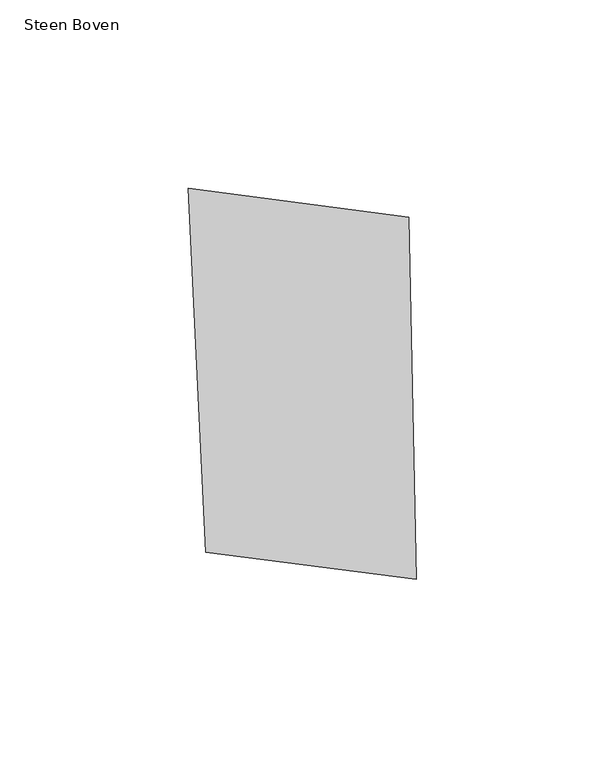
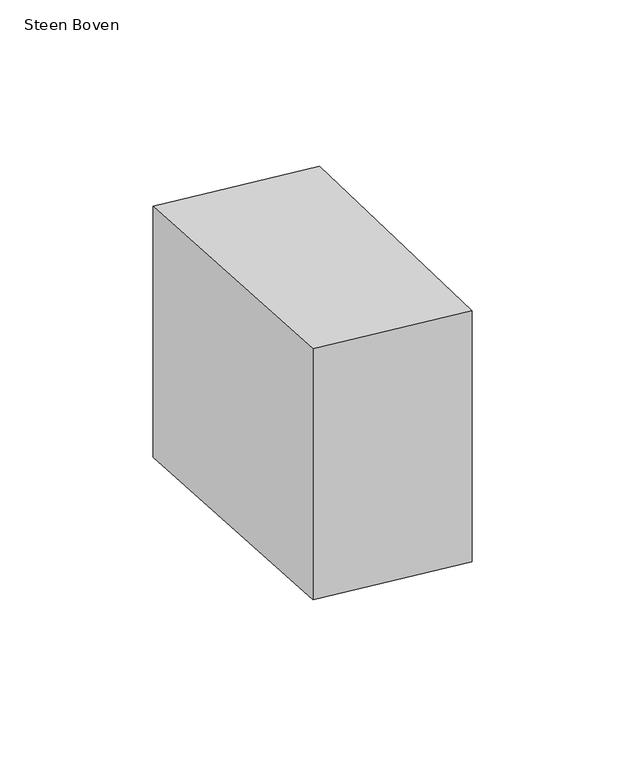
"""IFC4 building model written with IfcOpenShell, lengths in millimetres: proxy geometry, 00_GMA_steen_versie_4 : Steen Boven."""

from ifc_helpers import new_model, si_unit, origin, origin_with_axes, place, context, project, spatial, polyline, outline, extrude, source, transform, mapped, element, save


def steen_boven_6d589674(model_context):
    return source(origin(), model_context, "Body", "SweptSolid", [
        extrude(outline(polyline([(99.5503295, 119.8054673), (101.5366734, 23.6798931), (45.6696797, 30.9600241), (41.0816974, 127.4442682), (99.5503295, 119.8054673)])), origin_with_axes(), (0.0, 0.0, 1.0), 100.0),
    ])


if __name__ == "__main__":
    model = new_model("IFC4")
    model_context = context("Model", 3, world=origin())
    ifc_project = project(units=[si_unit("LENGTHUNIT", "METRE", prefix="MILLI")], contexts=[model_context])
    site = spatial("IfcSite", under=ifc_project)
    building = spatial("IfcBuilding", under=site)
    placement = place(None, origin())
    steen_boven_shape = steen_boven_6d589674(model_context)
    element("IfcBuildingElementProxy", 1, Name="00_GMA_steen_versie_4 : Steen Boven", ObjectType="00_GMA_steen_versie_4 : Steen Boven", at=placement, inside=building, context=model_context, shape_type="MappedRepresentation", body=[
        mapped(steen_boven_shape, transform((0.0, 0.0, 0.0), x_axis=(1.0, 0.0, 0.0), y_axis=(0.0, 1.0, 0.0), z_axis=(0.0, 0.0, 1.0))),
    ])
    save(model, "model.ifc")

# Revit data of these elements
# Type "00_GMA_steen_versie_4 : Steen Boven"
#   StootVoegHalfBoven [instance default] = 5 mm
#   StootVoegHalf [instance default] = 5 mm
#   StootVoegBreedteOnder = 10 mm
#   StootVoegBreedteBoven = 10 mm
#   Steendikte = 100 mm
#   LintVoegOnderHalf = 5 mm
#   LintVoegOnder = 10 mm
#   LintVoegBovenHalf = 0 mm
#   LintVoegBoven = 0 mm
#   materiaal = none
#   MateriaalVoeg = none
#   Default Elevation = 0
